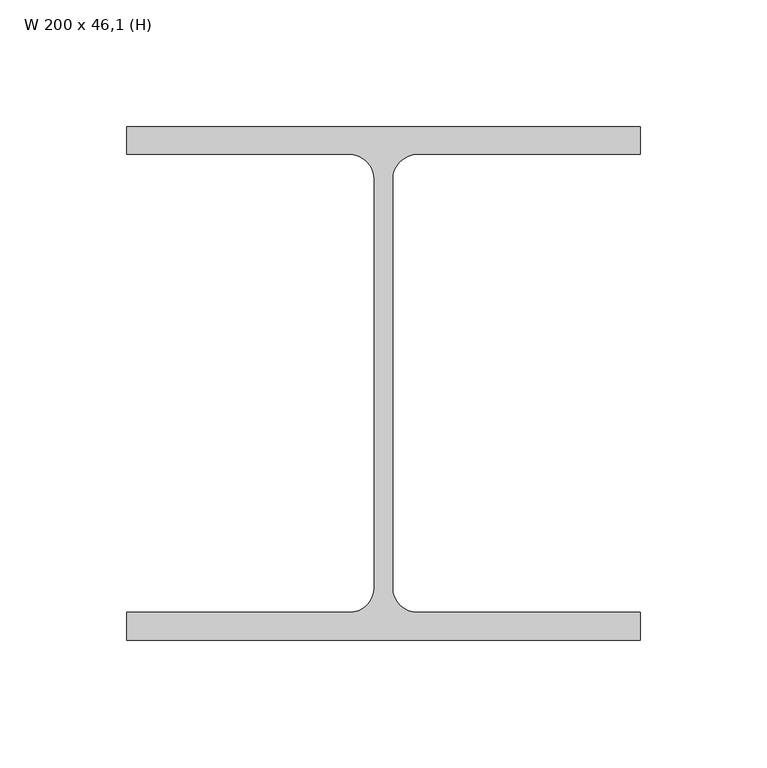
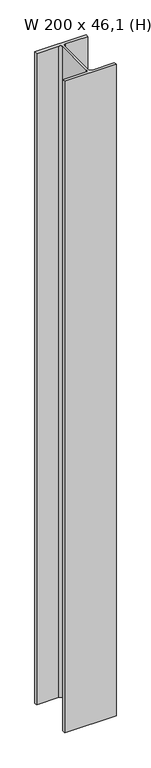
"""IFC4 building model written with IfcOpenShell, lengths in millimetres: column geometry, Pilar de Aço - H : W 200 x 46,1 (H)."""

from ifc_helpers import new_model, si_unit, point, frame_2d, origin, origin_with_axes, place, context, project, spatial, polyline, circle_curve, trimmed, segment, composite_curve, outline, extrude, source, transform, mapped, element, save


def w_200_x_46_1_h_d1e9d4fa(model_context):
    return source(origin(), model_context, "Body", "SweptSolid", [
        extrude(outline(composite_curve([segment(polyline([(101.5, 101.5), (101.5, 90.5), (13.6, 90.5)]), True, "CONTINUOUS"), segment(trimmed(circle_curve(frame_2d((13.6, 80.5)), 10.0), [point((13.6, 90.5))], [point((3.6, 80.5))], True, "CARTESIAN"), True, "CONTINUOUS"), segment(polyline([(3.6, 80.5), (3.6, -80.5)]), True, "CONTINUOUS"), segment(trimmed(circle_curve(frame_2d((13.6, -80.5)), 10.0), [point((3.6, -80.5))], [point((13.6, -90.5))], True, "CARTESIAN"), True, "CONTINUOUS"), segment(polyline([(13.6, -90.5), (101.5, -90.5), (101.5, -101.5), (-101.5, -101.5), (-101.5, -90.5), (-13.6, -90.5)]), True, "CONTINUOUS"), segment(trimmed(circle_curve(frame_2d((-13.6, -80.5)), 10.0), [point((-13.6, -90.5))], [point((-3.6, -80.5))], True, "CARTESIAN"), True, "CONTINUOUS"), segment(polyline([(-3.6, -80.5), (-3.6, 80.5)]), True, "CONTINUOUS"), segment(trimmed(circle_curve(frame_2d((-13.6, 80.5)), 10.0), [point((-3.6, 80.5))], [point((-13.6, 90.5))], True, "CARTESIAN"), True, "CONTINUOUS"), segment(polyline([(-13.6, 90.5), (-101.5, 90.5), (-101.5, 101.5), (101.5, 101.5)]), True, "CONTINUOUS")], self_intersect=False)), origin_with_axes(), (0.0, 0.0, 1.0), 2720.0),
    ])


if __name__ == "__main__":
    model = new_model("IFC4")
    model_context = context("Model", 3, world=origin())
    ifc_project = project(units=[si_unit("LENGTHUNIT", "METRE", prefix="MILLI")], contexts=[model_context])
    site = spatial("IfcSite", under=ifc_project)
    building = spatial("IfcBuilding", under=site)
    placement = place(None, origin())
    w_200_x_46_1_h_shape = w_200_x_46_1_h_d1e9d4fa(model_context)
    element("IfcColumn", 1, ObjectType="Pilar de Aço - H : W 200 x 46,1 (H)", at=placement, inside=building, context=model_context, shape_type="MappedRepresentation", body=[
        mapped(w_200_x_46_1_h_shape, transform((0.0, 0.0, 0.0), x_axis=(1.0, 0.0, 0.0), y_axis=(0.0, 1.0, 0.0), z_axis=(0.0, 0.0, 1.0))),
    ])
    save(model, "model.ifc")

# Revit data of these elements
# Type "Pilar de Aço - H : W 200 x 46,1 (H)"
#   SINAPI = ""
#   Área da seção = 56.6 m²
#   tw = 0.72 cm
#   tf = 1.10 cm
#   h = 18.10 cm
#   d' = 16.10 cm
#   d = 20.30 cm
#   bf = 20.30 cm
#   R = 1.00 cm
#   Massa Linear kg/m = 46.1
#   Aço = Metal - Aço 345MPa
#   Assembly Code = ""
# Materials
#   "Metal - Aço 345MPa": class "Metal", colour RGB 189 187 185, transparency 0, Cost = 0
